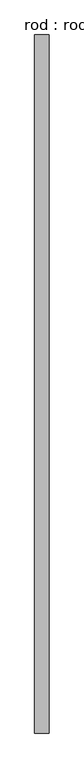
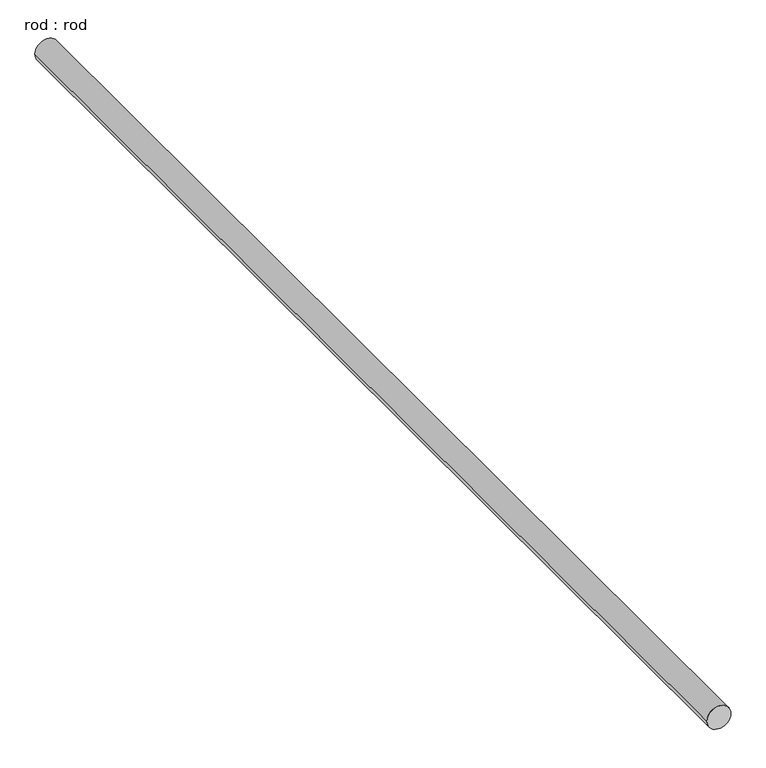
"""IFC4 building model written with IfcOpenShell, lengths in millimetres: proxy geometry, rod : rod."""

from ifc_helpers import new_model, si_unit, point, frame, frame_2d, origin, place, context, project, spatial, circle_curve, trimmed, segment, composite_curve, outline, extrude, source, transform, mapped, element, save


def rod_rod_63cc6917(model_context):
    return source(origin(), model_context, "Body", "SweptSolid", [
        extrude(outline(composite_curve([segment(trimmed(circle_curve(frame_2d((0.0108462, 0.0)), 200.0), [point((0.0108462, 200.0))], [point((0.0108462, -200.0))], False, "CARTESIAN"), True, "CONTINUOUS"), segment(trimmed(circle_curve(frame_2d((0.0108462, 0.0)), 200.0), [point((0.0108462, -200.0))], [point((0.0108462, 200.0))], False, "CARTESIAN"), True, "CONTINUOUS")], self_intersect=False)), frame((0.0, -5603.6999561, 0.0), z_axis=(0.0, 1.0, 0.0), x_axis=(0.0, 0.0, 1.0)), (0.0, 0.0, 1.0), 19392.8571429),
    ])


if __name__ == "__main__":
    model = new_model("IFC4")
    model_context = context("Model", 3, world=origin())
    ifc_project = project(units=[si_unit("LENGTHUNIT", "METRE", prefix="MILLI")], contexts=[model_context])
    site = spatial("IfcSite", under=ifc_project)
    building = spatial("IfcBuilding", under=site)
    placement = place(None, origin())
    rod_rod_shape = rod_rod_63cc6917(model_context)
    element("IfcBuildingElementProxy", 1, Name="rod : rod", ObjectType="rod : rod", at=placement, inside=building, context=model_context, shape_type="MappedRepresentation", body=[
        mapped(rod_rod_shape, transform((0.0, 0.0, 0.0), x_axis=(1.0, 0.0, 0.0), y_axis=(0.0, 1.0, 0.0), z_axis=(0.0, 0.0, 1.0))),
    ])
    save(model, "model.ifc")

# Revit data of these elements
# Type "rod : rod"
#   Default Elevation = 0
